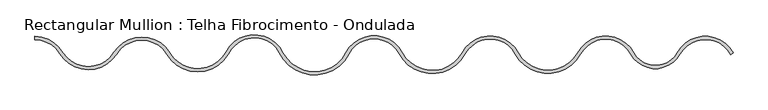
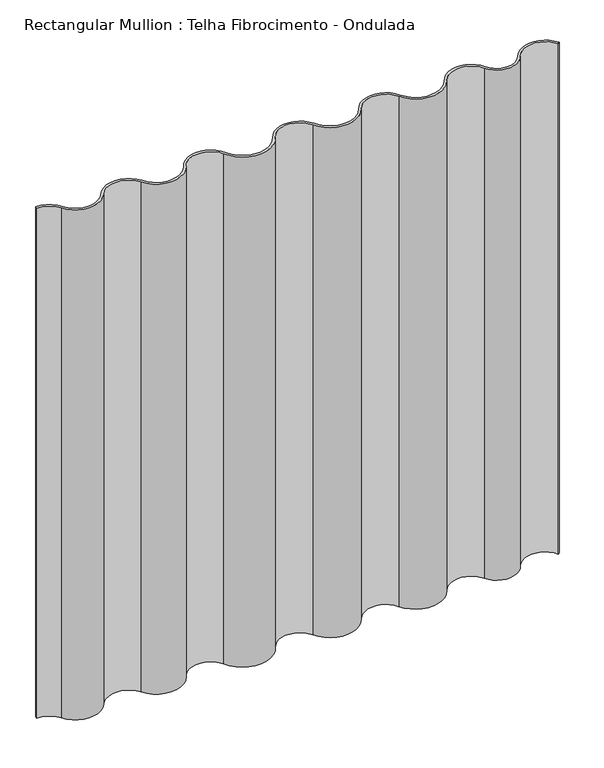
"""IFC4 building model written with IfcOpenShell, lengths in millimetres: member geometry, Rectangular Mullion : Telha Fibrocimento - Ondulada."""

from ifc_helpers import new_model, si_unit, point, frame, frame_2d, origin, place, context, project, spatial, polyline, circle_curve, trimmed, segment, composite_curve, outline, extrude, source, transform, mapped, element, save


def rectangular_mullion_telha_fibrocimento_ondulada_f148e399(model_context):
    return source(origin(), model_context, "Body", "SweptSolid", [
        extrude(outline(composite_curve([segment(trimmed(circle_curve(frame_2d((69.0116929, 0.1433824)), 54.0237163), [point((21.4619415, -25.5))], [point((116.5305219, -25.5572561))], True, "CARTESIAN"), True, "CONTINUOUS"), segment(trimmed(circle_curve(frame_2d((160.8849246, -49.5231629)), 50.4150545), [point((116.5305219, -25.5572561))], [point((205.2083424, -25.5))], False, "CARTESIAN"), True, "CONTINUOUS"), segment(trimmed(circle_curve(frame_2d((252.3825811, 0.1433824)), 53.6934993), [point((205.2083424, -25.5))], [point((299.4511352, -25.6934728))], True, "CARTESIAN"), True, "CONTINUOUS"), segment(trimmed(circle_curve(frame_2d((343.8078866, -50.0417661)), 50.6000078), [point((299.4511352, -25.6934728))], [point((388.0578866, -25.5))], False, "CARTESIAN"), True, "CONTINUOUS"), segment(trimmed(circle_curve(frame_2d((422.6668006, -6.5383891)), 39.4628891), [point((388.0578866, -25.5))], [point((457.2757147, -25.5))], True, "CARTESIAN"), True, "CONTINUOUS"), segment(trimmed(circle_curve(frame_2d((501.5257147, -50.5816659)), 50.8640587), [point((457.2757147, -25.5))], [point((545.7757147, -25.5))], False, "CARTESIAN"), True, "CONTINUOUS"), segment(polyline([(545.7757147, -25.5), (542.1028834, -29.2034416)]), True, "CONTINUOUS"), segment(trimmed(circle_curve(frame_2d((501.5257147, -50.5816659)), 45.8643118), [point((542.1028834, -29.2034416))], [point((461.6017876, -28.0070088))], True, "CARTESIAN"), True, "CONTINUOUS"), segment(trimmed(circle_curve(frame_2d((422.6668006, -6.5383891)), 44.4616109), [point((461.6017876, -28.0070088))], [point((383.7318137, -28.0070088))], False, "CARTESIAN"), True, "CONTINUOUS"), segment(trimmed(circle_curve(frame_2d((343.8078866, -50.0417661)), 45.6009921), [point((383.7318137, -28.0070088))], [point((303.8839595, -28.0070088))], True, "CARTESIAN"), True, "CONTINUOUS"), segment(trimmed(circle_curve(frame_2d((252.3825811, 0.1433824)), 58.6927295), [point((303.8839595, -28.0070088))], [point((200.8088517, -27.8742357))], False, "CARTESIAN"), True, "CONTINUOUS"), segment(trimmed(circle_curve(frame_2d((160.8849246, -49.5231629)), 45.4158123), [point((200.8088517, -27.8742357))], [point((120.8892858, -28.0070088))], True, "CARTESIAN"), True, "CONTINUOUS"), segment(trimmed(circle_curve(frame_2d((69.0116929, 0.1433824)), 59.023124), [point((120.8892858, -28.0070088))], [point((16.9239271, -27.6161893))], False, "CARTESIAN"), True, "CONTINUOUS"), segment(trimmed(circle_curve(frame_2d((-23.0, -49.053803)), 45.3154635), [point((16.9239271, -27.6161893))], [point((-63.1313306, -28.0070088))], True, "CARTESIAN"), True, "CONTINUOUS"), segment(trimmed(circle_curve(frame_2d((-117.4465095, 0.1433824)), 61.1766556), [point((-63.1313306, -28.0070088))], [point((-172.9665492, -25.5491921))], False, "CARTESIAN"), True, "CONTINUOUS"), segment(trimmed(circle_curve(frame_2d((-212.8904763, -48.1747621)), 45.8893928), [point((-172.9665492, -25.5491921))], [point((-254.110594, -28.0070088))], True, "CARTESIAN"), True, "CONTINUOUS"), segment(trimmed(circle_curve(frame_2d((-302.659059, 0.1433824)), 56.1194973), [point((-254.110594, -28.0070088))], [point((-351.2075239, -28.0070088))], False, "CARTESIAN"), True, "CONTINUOUS"), segment(trimmed(circle_curve(frame_2d((-391.131451, -52.953971)), 47.0772862), [point((-351.2075239, -28.0070088))], [point((-431.0553781, -28.0070088))], True, "CARTESIAN"), True, "CONTINUOUS"), segment(trimmed(circle_curve(frame_2d((-475.7915893, 0.1433824)), 52.8561549), [point((-431.0553781, -28.0070088))], [point((-521.0773689, -27.114117))], False, "CARTESIAN"), True, "CONTINUOUS"), segment(trimmed(circle_curve(frame_2d((-560.4742853, -51.1369128)), 46.1433824), [point((-521.0773689, -27.114117))], [point((-560.4742853, -4.9935304))], True, "CARTESIAN"), True, "CONTINUOUS"), segment(polyline([(-560.4742853, -4.9935304), (-560.4742853, 0.0)]), True, "CONTINUOUS"), segment(trimmed(circle_curve(frame_2d((-560.4742853, -51.1369128)), 51.1369128), [point((-560.4742853, 0.0))], [point((-516.2280137, -25.5))], False, "CARTESIAN"), True, "CONTINUOUS"), segment(trimmed(circle_curve(frame_2d((-475.7915893, 0.1433824)), 47.8820163), [point((-516.2280137, -25.5))], [point((-435.2460411, -25.3271104))], True, "CARTESIAN"), True, "CONTINUOUS"), segment(trimmed(circle_curve(frame_2d((-391.131451, -52.953971)), 52.0513254), [point((-435.2460411, -25.3271104))], [point((-346.909059, -25.5))], False, "CARTESIAN"), True, "CONTINUOUS"), segment(trimmed(circle_curve(frame_2d((-302.659059, 0.1433824)), 51.1433824), [point((-346.909059, -25.5))], [point((-257.6416121, -24.1274857))], True, "CARTESIAN"), True, "CONTINUOUS"), segment(trimmed(circle_curve(frame_2d((-212.8904763, -48.1747621)), 50.8029099), [point((-257.6416121, -24.1274857))], [point((-167.4285052, -25.5))], False, "CARTESIAN"), True, "CONTINUOUS"), segment(trimmed(circle_curve(frame_2d((-117.4465095, 0.1433824)), 56.1763558), [point((-167.4285052, -25.5))], [point((-67.6156919, -25.7925495))], True, "CARTESIAN"), True, "CONTINUOUS"), segment(trimmed(circle_curve(frame_2d((-23.0, -49.053803)), 50.3154635), [point((-67.6156919, -25.7925495))], [point((21.4619415, -25.5))], False, "CARTESIAN"), True, "CONTINUOUS")], self_intersect=False)), frame((0.0, 0.0, -1154.7005384), z_axis=(0.0, 0.0, 1.0), x_axis=(1.0, 0.0, 0.0)), (0.0, 0.0, 1.0), 1154.7005384),
    ])


if __name__ == "__main__":
    model = new_model("IFC4")
    model_context = context("Model", 3, world=origin())
    ifc_project = project(units=[si_unit("LENGTHUNIT", "METRE", prefix="MILLI")], contexts=[model_context])
    site = spatial("IfcSite", under=ifc_project)
    building = spatial("IfcBuilding", under=site)
    placement = place(None, origin())
    rectangular_mullion_telha_fibrocimento_ondulada_shape = rectangular_mullion_telha_fibrocimento_ondulada_f148e399(model_context)
    element("IfcMember", 1, ObjectType="Rectangular Mullion : Telha Fibrocimento - Ondulada", at=placement, inside=building, context=model_context, shape_type="MappedRepresentation", body=[
        mapped(rectangular_mullion_telha_fibrocimento_ondulada_shape, transform((0.0, 0.0, 0.0), x_axis=(1.0, 0.0, 0.0), y_axis=(0.0, 1.0, 0.0), z_axis=(0.0, 0.0, 1.0))),
    ])
    save(model, "model.ifc")

# Revit data of these elements
# Type "Rectangular Mullion : Telha Fibrocimento - Ondulada"
#   built-in parameter 1007322 = 0.0284047 (stored number, unit not read)
#   built-in parameter 1007321 = 1.66299 (stored number, unit not read)
#   built-in parameter 1007320 = 1.83883 (stored number, unit not read)
# Element 1 (IfcMember, "Rectangular Mullion : Telha Fibrocimento - Ondulada")
#   Materials on its faces: "Telha - Fibrocimento"
# Materials
#   "Telha - Fibrocimento": class "Cimento", colour RGB 77 77 76, transparency 0, Cost = 0
